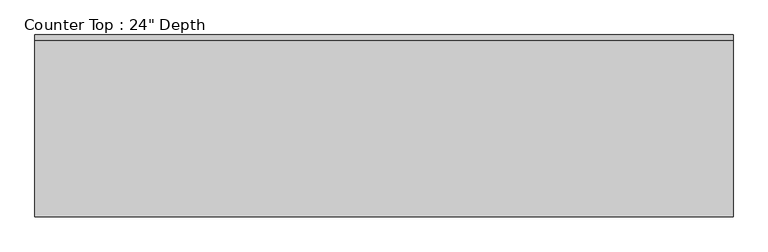
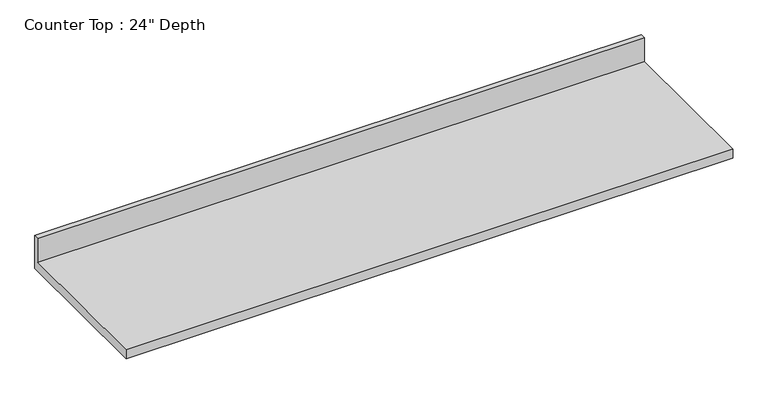
"""IFC4 building model written with IfcOpenShell, lengths in millimetres: furniture geometry."""

import ifcopenshell
import ifcopenshell.guid

model = None  # the IFC model being written
_history = None  # IfcOwnerHistory: only IFC2X3 demands one
_inside = {}  # id of a spatial element -> (the spatial element, [elements in it])
_under = {}  # id of a project, library or spatial element -> (it, [spatial elements below it])
_declared = {}  # id of a project -> (the project, [libraries it declares])
_typed = {}  # id of a type object -> (the type object, [elements of that type])
_made_of = {}  # id of a material, layer set ... -> (it, [elements and type objects made of it])


def new_model(schema):
    """Start an empty IFC model of exactly this schema.

    Asked for "IFC4X3", IfcOpenShell would pick the latest addendum, in which some entities
    have other attributes; the version numbers below select the first issue.
    IFC2X3 requires an IfcOwnerHistory on every rooted entity: one is made here for all.
    """
    global model, _history
    if schema == "IFC4X3":
        model = ifcopenshell.file(schema_version=(4, 3, 0, 0))
    else:
        model = ifcopenshell.file(schema=schema)
    _inside.clear()
    _under.clear()
    _declared.clear()
    _typed.clear()
    _made_of.clear()
    _history = None
    if model.schema == "IFC2X3":
        org = make("IfcOrganization", Name="unknown")
        user = make(
            "IfcPersonAndOrganization",
            ThePerson=make("IfcPerson", FamilyName="unknown"),
            TheOrganization=org,
        )
        app = make(
            "IfcApplication",
            ApplicationDeveloper=org,
            Version="unknown",
            ApplicationFullName="unknown",
            ApplicationIdentifier="unknown",
        )
        _history = make(
            "IfcOwnerHistory",
            OwningUser=user,
            OwningApplication=app,
            ChangeAction="ADDED",
            CreationDate=0,
        )
    return model


def make(cls, **values):
    """One entity of the class cls with the attributes given. An attribute that is None is left unset."""
    return model.create_entity(
        cls, **{name: value for name, value in values.items() if value is not None}
    )


def rooted(cls, **values):
    """An entity with a GlobalId (a new one), such as an element, a storey or a relation."""
    return make(cls, GlobalId=ifcopenshell.guid.new(), OwnerHistory=_history, **values)


def si_unit(unit_type, name, prefix=None):
    """IfcSIUnit, for example si_unit("LENGTHUNIT", "METRE", prefix="MILLI")."""
    return make("IfcSIUnit", UnitType=unit_type, Prefix=prefix, Name=name)


def assignment(units):
    """IfcUnitAssignment: the units of a project."""
    return None if units is None else make("IfcUnitAssignment", Units=units)


def point(xyz):
    """IfcCartesianPoint."""
    return None if xyz is None else make("IfcCartesianPoint", Coordinates=xyz)


def direction(xyz):
    """IfcDirection."""
    return None if xyz is None else make("IfcDirection", DirectionRatios=xyz)


def frame(location, z_axis=None, x_axis=None):
    """IfcAxis2Placement3D, a coordinate frame: its origin and axes. An axis left out is left unset."""
    return make(
        "IfcAxis2Placement3D",
        Location=point(location),
        Axis=direction(z_axis),
        RefDirection=direction(x_axis),
    )


def origin():
    """The frame at (0, 0, 0) with its axes left unset."""
    return frame((0.0, 0.0, 0.0))


def place(relative_to, where):
    """IfcLocalPlacement: puts the frame where relative to a parent placement (None: the world)."""
    return make(
        "IfcLocalPlacement", PlacementRelTo=relative_to, RelativePlacement=where
    )


def context(
    kind, dimensions, precision=None, world=None, true_north=None, identifier=None
):
    """IfcGeometricRepresentationContext, for example the 3D "Model" context."""
    return make(
        "IfcGeometricRepresentationContext",
        ContextIdentifier=identifier,
        ContextType=kind,
        CoordinateSpaceDimension=dimensions,
        Precision=precision,
        WorldCoordinateSystem=world,
        TrueNorth=true_north,
    )


def project(units=None, contexts=None):
    """IfcProject with its units and contexts."""
    return rooted(
        "IfcProject",
        Name="project",
        RepresentationContexts=contexts,
        UnitsInContext=assignment(units),
    )


def spatial(cls, under=None, at=None, **own):
    """A site, building, storey or space (cls), placed at a placement, below another one or the project."""
    s = rooted(cls, ObjectPlacement=at, **own)
    if under is not None:
        _under.setdefault(under.id(), (under, []))[1].append(s)
    return s


def polyline(points):
    """IfcPolyline through the points."""
    return make("IfcPolyline", Points=[point(p) for p in points])


def outline(outer, holes=None, kind="AREA"):
    """IfcArbitraryClosedProfileDef: a profile drawn as a closed curve; with holes, ...WithVoids."""
    if holes is None:
        return make("IfcArbitraryClosedProfileDef", ProfileType=kind, OuterCurve=outer)
    return make(
        "IfcArbitraryProfileDefWithVoids",
        ProfileType=kind,
        OuterCurve=outer,
        InnerCurves=holes,
    )


def extrude(swept, where, along, depth):
    """IfcExtrudedAreaSolid: the profile swept, set in the frame where, extruded along a direction by depth."""
    return make(
        "IfcExtrudedAreaSolid",
        SweptArea=swept,
        Position=where,
        ExtrudedDirection=direction(along),
        Depth=depth,
    )


def shape(context_of_items, identifier, shape_type, items):
    """IfcShapeRepresentation: the items that make up one representation, for example the "Body"."""
    return make(
        "IfcShapeRepresentation",
        ContextOfItems=context_of_items,
        RepresentationIdentifier=identifier,
        RepresentationType=shape_type,
        Items=items,
    )


def source(mapping_origin, context_of_items, identifier, shape_type, items):
    """IfcRepresentationMap: a shape defined once, which mapped items show again and again."""
    return make(
        "IfcRepresentationMap",
        MappingOrigin=mapping_origin,
        MappedRepresentation=shape(context_of_items, identifier, shape_type, items),
    )


def transform(
    local_origin,
    x_axis=None,
    y_axis=None,
    z_axis=None,
    scale=None,
    scale2=None,
    scale3=None,
    uniform=True,
):
    """IfcCartesianTransformationOperator3D, or its non-uniform kind. x_axis, y_axis, z_axis: its Axis1, 2, 3."""
    if uniform:
        return make(
            "IfcCartesianTransformationOperator3D",
            Axis1=direction(x_axis),
            Axis2=direction(y_axis),
            LocalOrigin=point(local_origin),
            Scale=scale,
            Axis3=direction(z_axis),
        )
    return make(
        "IfcCartesianTransformationOperator3DnonUniform",
        Axis1=direction(x_axis),
        Axis2=direction(y_axis),
        LocalOrigin=point(local_origin),
        Scale=scale,
        Axis3=direction(z_axis),
        Scale2=scale2,
        Scale3=scale3,
    )


def mapped(mapping_source, mapping_target):
    """IfcMappedItem: shows the shape of a source again, moved by a transform."""
    return make(
        "IfcMappedItem", MappingSource=mapping_source, MappingTarget=mapping_target
    )


def made_of(thing, what):
    """Note that an element or type object is made of a material, layer set ...; save() writes the relation."""
    if what is not None:
        _made_of.setdefault(what.id(), (what, []))[1].append(thing)
    return thing


def element(
    cls,
    number,
    at=None,
    inside=None,
    cuts=None,
    type_object=None,
    material=None,
    context=None,
    identifier="Body",
    shape_type=None,
    held_by="IfcProductDefinitionShape",
    body=None,
    shapes=None,
    **own,
):
    """One element of the class cls, such as IfcWall. Its Tag is "e" and its number.

    at: its placement. inside: the storey or other place that contains it. cuts: it is an
    opening in that element (IfcRelVoidsElement). A single representation is given by context,
    identifier, shape_type and body (its items); several are given by shapes. held_by: the class
    of the entity that holds the representations. save() writes the other relations.
    """
    e = rooted(cls, Tag="e%d" % number, ObjectPlacement=at, **own)
    if body is not None:
        shapes = [shape(context, identifier, shape_type, body)]
    if shapes is not None:
        e.Representation = make(held_by, Representations=shapes)
    if inside is not None:
        _inside.setdefault(inside.id(), (inside, []))[1].append(e)
    if cuts is not None:
        rooted(
            "IfcRelVoidsElement", RelatingBuildingElement=cuts, RelatedOpeningElement=e
        )
    if type_object is not None:
        _typed.setdefault(type_object.id(), (type_object, []))[1].append(e)
    return made_of(e, material)


def aggregate(whole, parts):
    """IfcRelAggregates: a whole, such as a stair, and the parts it consists of."""
    return rooted("IfcRelAggregates", RelatingObject=whole, RelatedObjects=parts)


def save(model, path):
    """Write the relations noted so far, then the file.

    IfcRelAggregates (storeys below a building ...), IfcRelContainedInSpatialStructure (elements
    in a storey), IfcRelDefinesByType, IfcRelAssociatesMaterial and IfcRelDeclares: one each for
    every whole, place, type object, material and project.
    """
    for whole, parts in _under.values():
        aggregate(whole, parts)
    for where, things in _inside.values():
        rooted(
            "IfcRelContainedInSpatialStructure",
            RelatedElements=things,
            RelatingStructure=where,
        )
    for kind, things in _typed.values():
        rooted("IfcRelDefinesByType", RelatedObjects=things, RelatingType=kind)
    for what, things in _made_of.values():
        rooted("IfcRelAssociatesMaterial", RelatedObjects=things, RelatingMaterial=what)
    for by, libraries in _declared.values():
        rooted("IfcRelDeclares", RelatingContext=by, RelatedDefinitions=libraries)
    model.write(path)


def furniture_deb1c5d1(model_context):
    return source(origin(), model_context, "Body", "SweptSolid", [
        extrude(outline(polyline([(0.0, 1016.0), (0.0, 876.3), (-635.0, 876.3), (-635.0, 914.4), (-19.05, 914.4), (-19.05, 1016.0), (0.0, 1016.0)])), frame((-1200.4622951, 0.0, 0.0), z_axis=(1.0, 0.0, 0.0), x_axis=(0.0, 1.0, 0.0)), (0.0, 0.0, 1.0), 2438.4),
    ])


if __name__ == "__main__":
    model = new_model("IFC4")
    model_context = context("Model", 3, world=origin())
    ifc_project = project(units=[si_unit("LENGTHUNIT", "METRE", prefix="MILLI")], contexts=[model_context])
    site = spatial("IfcSite", under=ifc_project)
    building = spatial("IfcBuilding", under=site)
    placement = place(None, origin())
    furniture_shape = furniture_deb1c5d1(model_context)
    element("IfcFurniture", 1, ObjectType="Counter Top : 24\" Depth", at=placement, inside=building, context=model_context, shape_type="MappedRepresentation", body=[
        mapped(furniture_shape, transform((0.0, 0.0, 0.0), x_axis=(1.0, 0.0, 0.0), y_axis=(0.0, 1.0, 0.0), z_axis=(0.0, 0.0, 1.0))),
    ])
    save(model, "model.ifc")

# Revit data of these elements
# Type "Counter Top : 24\" Depth"
#   Assembly Code = "C1030400"
#   Counter Thickness = 0' - 1 1/2"
#   Depth = 2' - 1"
#   Height = 3' - 0"
#   Length [instance default] = 8' - 0"
#   Counter Top Material = none
#   Default Elevation = 0
# Element 1 (IfcFurniture, "Counter Top : 24\" Depth")
#   Materials on its faces: "Counter Top"
# Materials
#   "Counter Top": class "Wood", colour RGB 226 177 128, transparency 0, Cost = 0
